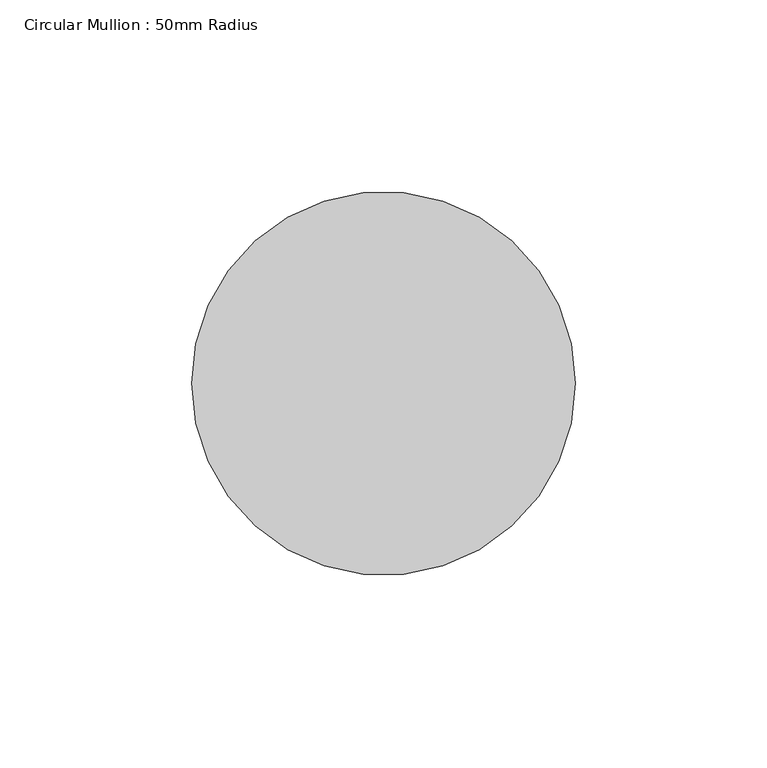
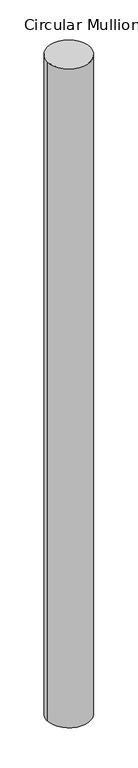
"""IFC4 building model written with IfcOpenShell, lengths in millimetres: member geometry, Circular Mullion : 50mm Radius."""

from ifc_helpers import new_model, si_unit, point, frame, origin, origin_2d, place, context, project, spatial, circle_curve, trimmed, segment, composite_curve, outline, extrude, source, transform, mapped, element, save


def circular_mullion_50mm_radius_b5959d2e(model_context):
    return source(origin(), model_context, "Body", "SweptSolid", [
        extrude(outline(composite_curve([segment(trimmed(circle_curve(origin_2d(), 50.0), [point((50.0, 0.0))], [point((-50.0, 0.0))], False, "CARTESIAN"), True, "CONTINUOUS"), segment(trimmed(circle_curve(origin_2d(), 50.0), [point((-50.0, 0.0))], [point((50.0, 0.0))], False, "CARTESIAN"), True, "CONTINUOUS")], self_intersect=False)), frame((0.0, 0.0, -1609.5880264), z_axis=(0.0, 0.0, 1.0), x_axis=(1.0, 0.0, 0.0)), (0.0, 0.0, 1.0), 1609.5880264),
    ])


if __name__ == "__main__":
    model = new_model("IFC4")
    model_context = context("Model", 3, world=origin())
    ifc_project = project(units=[si_unit("LENGTHUNIT", "METRE", prefix="MILLI")], contexts=[model_context])
    site = spatial("IfcSite", under=ifc_project)
    building = spatial("IfcBuilding", under=site)
    placement = place(None, origin())
    circular_mullion_50mm_radius_shape = circular_mullion_50mm_radius_b5959d2e(model_context)
    element("IfcMember", 1, ObjectType="Circular Mullion : 50mm Radius", at=placement, inside=building, context=model_context, shape_type="MappedRepresentation", body=[
        mapped(circular_mullion_50mm_radius_shape, transform((0.0, 0.0, 0.0), x_axis=(1.0, 0.0, 0.0), y_axis=(0.0, 1.0, 0.0), z_axis=(0.0, 0.0, 1.0))),
    ])
    save(model, "model.ifc")

# Revit data of these elements
# Type "Circular Mullion : 50mm Radius"
#   built-in parameter 1007350 = 0.164042 (stored number, unit not read)
# Element 1 (IfcMember, "Circular Mullion : 50mm Radius")
#   Materials on its faces: "Aluminium"
# Materials
#   "Aluminium": class "Metal", colour RGB 247 247 247, transparency 0, Description = "Aluminium 6061", Cost = 0
